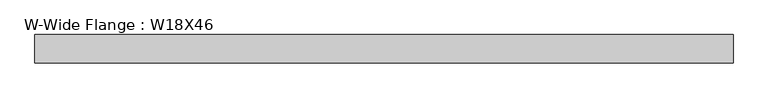
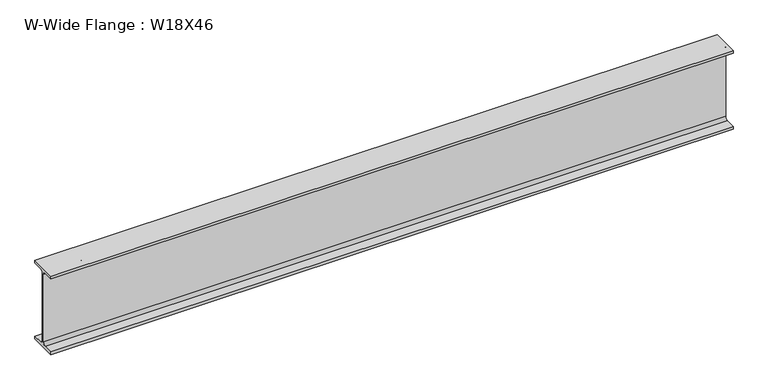
"""IFC4 building model written with IfcOpenShell, lengths in millimetres: beam geometry, W-Wide Flange : W18X46."""

from ifc_helpers import new_model, si_unit, point, frame, frame_2d, origin, place, context, project, spatial, polyline, circle_curve, trimmed, segment, composite_curve, outline, extrude, source, transform, mapped, element, save


def w_wide_flange_w18x46_cc853d8d(model_context):
    return source(origin(), model_context, "Body", "SweptSolid", [
        extrude(outline(composite_curve([segment(polyline([(76.962, -214.503), (76.962, -229.87), (-76.962, -229.87), (-76.962, -214.503), (-20.955, -214.503)]), True, "CONTINUOUS"), segment(trimmed(circle_curve(frame_2d((-20.955, -198.12)), 16.383), [point((-20.955, -214.503))], [point((-4.572, -198.12))], True, "CARTESIAN"), True, "CONTINUOUS"), segment(polyline([(-4.572, -198.12), (-4.572, 198.12)]), True, "CONTINUOUS"), segment(trimmed(circle_curve(frame_2d((-20.955, 198.12)), 16.383), [point((-4.572, 198.12))], [point((-20.955, 214.503))], True, "CARTESIAN"), True, "CONTINUOUS"), segment(polyline([(-20.955, 214.503), (-76.962, 214.503), (-76.962, 229.87), (76.962, 229.87), (76.962, 214.503), (20.955, 214.503)]), True, "CONTINUOUS"), segment(trimmed(circle_curve(frame_2d((20.955, 198.12)), 16.383), [point((20.955, 214.503))], [point((4.572, 198.12))], True, "CARTESIAN"), True, "CONTINUOUS"), segment(polyline([(4.572, 198.12), (4.572, -198.12)]), True, "CONTINUOUS"), segment(trimmed(circle_curve(frame_2d((20.955, -198.12)), 16.383), [point((4.572, -198.12))], [point((20.955, -214.503))], True, "CARTESIAN"), True, "CONTINUOUS"), segment(polyline([(20.955, -214.503), (76.962, -214.503)]), True, "CONTINUOUS")], self_intersect=False)), frame((-1892.3, 0.0, 0.0), z_axis=(1.0, 0.0, 0.0), x_axis=(0.0, 1.0, 0.0)), (0.0, 0.0, 1.0), 3784.6),
    ])


if __name__ == "__main__":
    model = new_model("IFC4")
    model_context = context("Model", 3, world=origin())
    ifc_project = project(units=[si_unit("LENGTHUNIT", "METRE", prefix="MILLI")], contexts=[model_context])
    site = spatial("IfcSite", under=ifc_project)
    building = spatial("IfcBuilding", under=site)
    placement = place(None, origin())
    w_wide_flange_w18x46_shape = w_wide_flange_w18x46_cc853d8d(model_context)
    element("IfcBeam", 1, ObjectType="W-Wide Flange : W18X46", at=placement, inside=building, context=model_context, shape_type="MappedRepresentation", body=[
        mapped(w_wide_flange_w18x46_shape, transform((0.0, 0.0, 0.0), x_axis=(1.0, 0.0, 0.0), y_axis=(0.0, 1.0, 0.0), z_axis=(0.0, 0.0, 1.0))),
    ])
    save(model, "model.ifc")

# Revit data of these elements
# Type "W-Wide Flange : W18X46"
#   Assembly Code = "B10"
#   W = 46
#   Length [instance default] = 5' - 0"
#   bf = 0' - 6.06"
#   d = 1' - 6.1"
#   k = 0' - 1 1/4"
#   k2 = 0' - 0.645"
#   tf = 0' - 0.605"
#   tw = 0' - 0.36"
#   A = 0.09375 SF
#   Structural Material [instance default] = Steel ASTM A992
# Element 1 (IfcBeam, "W-Wide Flange : W18X46")
#   Materials on its faces: "Steel ASTM A992"
# Materials
#   "Steel ASTM A992": class "Metal", colour RGB 199 199 199, transparency 0, Description = "Structural steel 50ksi", Cost = 0
